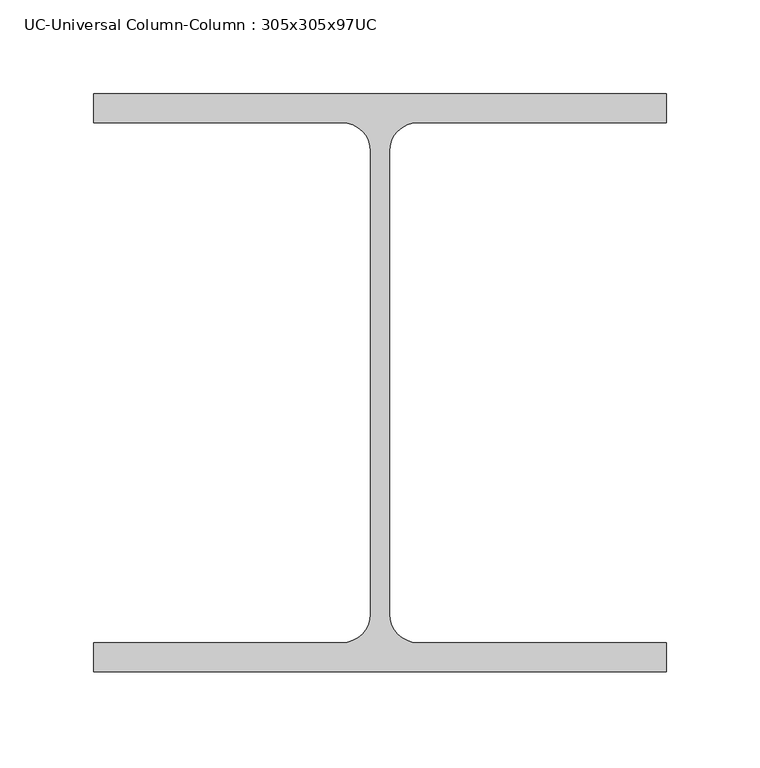
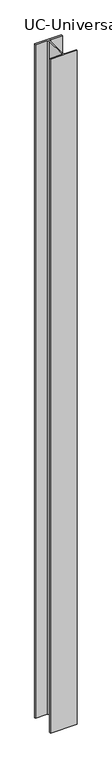
"""IFC4 building model written with IfcOpenShell, lengths in millimetres: column geometry, UC-Universal Column-Column : 305x305x97UC."""

import ifcopenshell
import ifcopenshell.guid

model = None  # the IFC model being written
_history = None  # IfcOwnerHistory: only IFC2X3 demands one
_inside = {}  # id of a spatial element -> (the spatial element, [elements in it])
_under = {}  # id of a project, library or spatial element -> (it, [spatial elements below it])
_declared = {}  # id of a project -> (the project, [libraries it declares])
_typed = {}  # id of a type object -> (the type object, [elements of that type])
_made_of = {}  # id of a material, layer set ... -> (it, [elements and type objects made of it])


def new_model(schema):
    """Start an empty IFC model of exactly this schema.

    Asked for "IFC4X3", IfcOpenShell would pick the latest addendum, in which some entities
    have other attributes; the version numbers below select the first issue.
    IFC2X3 requires an IfcOwnerHistory on every rooted entity: one is made here for all.
    """
    global model, _history
    if schema == "IFC4X3":
        model = ifcopenshell.file(schema_version=(4, 3, 0, 0))
    else:
        model = ifcopenshell.file(schema=schema)
    _inside.clear()
    _under.clear()
    _declared.clear()
    _typed.clear()
    _made_of.clear()
    _history = None
    if model.schema == "IFC2X3":
        org = make("IfcOrganization", Name="unknown")
        user = make(
            "IfcPersonAndOrganization",
            ThePerson=make("IfcPerson", FamilyName="unknown"),
            TheOrganization=org,
        )
        app = make(
            "IfcApplication",
            ApplicationDeveloper=org,
            Version="unknown",
            ApplicationFullName="unknown",
            ApplicationIdentifier="unknown",
        )
        _history = make(
            "IfcOwnerHistory",
            OwningUser=user,
            OwningApplication=app,
            ChangeAction="ADDED",
            CreationDate=0,
        )
    return model


def make(cls, **values):
    """One entity of the class cls with the attributes given. An attribute that is None is left unset."""
    return model.create_entity(
        cls, **{name: value for name, value in values.items() if value is not None}
    )


def rooted(cls, **values):
    """An entity with a GlobalId (a new one), such as an element, a storey or a relation."""
    return make(cls, GlobalId=ifcopenshell.guid.new(), OwnerHistory=_history, **values)


def si_unit(unit_type, name, prefix=None):
    """IfcSIUnit, for example si_unit("LENGTHUNIT", "METRE", prefix="MILLI")."""
    return make("IfcSIUnit", UnitType=unit_type, Prefix=prefix, Name=name)


def assignment(units):
    """IfcUnitAssignment: the units of a project."""
    return None if units is None else make("IfcUnitAssignment", Units=units)


def point(xyz):
    """IfcCartesianPoint."""
    return None if xyz is None else make("IfcCartesianPoint", Coordinates=xyz)


def direction(xyz):
    """IfcDirection."""
    return None if xyz is None else make("IfcDirection", DirectionRatios=xyz)


def frame(location, z_axis=None, x_axis=None):
    """IfcAxis2Placement3D, a coordinate frame: its origin and axes. An axis left out is left unset."""
    return make(
        "IfcAxis2Placement3D",
        Location=point(location),
        Axis=direction(z_axis),
        RefDirection=direction(x_axis),
    )


def frame_2d(location, x_axis=None):
    """IfcAxis2Placement2D, a coordinate frame in the plane: its origin and x axis."""
    return make(
        "IfcAxis2Placement2D", Location=point(location), RefDirection=direction(x_axis)
    )


def origin():
    """The frame at (0, 0, 0) with its axes left unset."""
    return frame((0.0, 0.0, 0.0))


def place(relative_to, where):
    """IfcLocalPlacement: puts the frame where relative to a parent placement (None: the world)."""
    return make(
        "IfcLocalPlacement", PlacementRelTo=relative_to, RelativePlacement=where
    )


def context(
    kind, dimensions, precision=None, world=None, true_north=None, identifier=None
):
    """IfcGeometricRepresentationContext, for example the 3D "Model" context."""
    return make(
        "IfcGeometricRepresentationContext",
        ContextIdentifier=identifier,
        ContextType=kind,
        CoordinateSpaceDimension=dimensions,
        Precision=precision,
        WorldCoordinateSystem=world,
        TrueNorth=true_north,
    )


def project(units=None, contexts=None):
    """IfcProject with its units and contexts."""
    return rooted(
        "IfcProject",
        Name="project",
        RepresentationContexts=contexts,
        UnitsInContext=assignment(units),
    )


def spatial(cls, under=None, at=None, **own):
    """A site, building, storey or space (cls), placed at a placement, below another one or the project."""
    s = rooted(cls, ObjectPlacement=at, **own)
    if under is not None:
        _under.setdefault(under.id(), (under, []))[1].append(s)
    return s


def polyline(points):
    """IfcPolyline through the points."""
    return make("IfcPolyline", Points=[point(p) for p in points])


def circle_curve(where, radius):
    """IfcCircle in the frame where."""
    return make("IfcCircle", Position=where, Radius=radius)


def trimmed(basis, trim1, trim2, sense, master):
    """IfcTrimmedCurve: the piece of a basis curve between two trims."""
    return make(
        "IfcTrimmedCurve",
        BasisCurve=basis,
        Trim1=trim1,
        Trim2=trim2,
        SenseAgreement=sense,
        MasterRepresentation=master,
    )


def segment(curve, same_sense, transition):
    """IfcCompositeCurveSegment."""
    return make(
        "IfcCompositeCurveSegment",
        Transition=transition,
        SameSense=same_sense,
        ParentCurve=curve,
    )


def composite_curve(segments, self_intersect=None):
    """IfcCompositeCurve: segments joined end to end."""
    return make("IfcCompositeCurve", Segments=segments, SelfIntersect=self_intersect)


def outline(outer, holes=None, kind="AREA"):
    """IfcArbitraryClosedProfileDef: a profile drawn as a closed curve; with holes, ...WithVoids."""
    if holes is None:
        return make("IfcArbitraryClosedProfileDef", ProfileType=kind, OuterCurve=outer)
    return make(
        "IfcArbitraryProfileDefWithVoids",
        ProfileType=kind,
        OuterCurve=outer,
        InnerCurves=holes,
    )


def extrude(swept, where, along, depth):
    """IfcExtrudedAreaSolid: the profile swept, set in the frame where, extruded along a direction by depth."""
    return make(
        "IfcExtrudedAreaSolid",
        SweptArea=swept,
        Position=where,
        ExtrudedDirection=direction(along),
        Depth=depth,
    )


def shape(context_of_items, identifier, shape_type, items):
    """IfcShapeRepresentation: the items that make up one representation, for example the "Body"."""
    return make(
        "IfcShapeRepresentation",
        ContextOfItems=context_of_items,
        RepresentationIdentifier=identifier,
        RepresentationType=shape_type,
        Items=items,
    )


def source(mapping_origin, context_of_items, identifier, shape_type, items):
    """IfcRepresentationMap: a shape defined once, which mapped items show again and again."""
    return make(
        "IfcRepresentationMap",
        MappingOrigin=mapping_origin,
        MappedRepresentation=shape(context_of_items, identifier, shape_type, items),
    )


def transform(
    local_origin,
    x_axis=None,
    y_axis=None,
    z_axis=None,
    scale=None,
    scale2=None,
    scale3=None,
    uniform=True,
):
    """IfcCartesianTransformationOperator3D, or its non-uniform kind. x_axis, y_axis, z_axis: its Axis1, 2, 3."""
    if uniform:
        return make(
            "IfcCartesianTransformationOperator3D",
            Axis1=direction(x_axis),
            Axis2=direction(y_axis),
            LocalOrigin=point(local_origin),
            Scale=scale,
            Axis3=direction(z_axis),
        )
    return make(
        "IfcCartesianTransformationOperator3DnonUniform",
        Axis1=direction(x_axis),
        Axis2=direction(y_axis),
        LocalOrigin=point(local_origin),
        Scale=scale,
        Axis3=direction(z_axis),
        Scale2=scale2,
        Scale3=scale3,
    )


def mapped(mapping_source, mapping_target):
    """IfcMappedItem: shows the shape of a source again, moved by a transform."""
    return make(
        "IfcMappedItem", MappingSource=mapping_source, MappingTarget=mapping_target
    )


def made_of(thing, what):
    """Note that an element or type object is made of a material, layer set ...; save() writes the relation."""
    if what is not None:
        _made_of.setdefault(what.id(), (what, []))[1].append(thing)
    return thing


def element(
    cls,
    number,
    at=None,
    inside=None,
    cuts=None,
    type_object=None,
    material=None,
    context=None,
    identifier="Body",
    shape_type=None,
    held_by="IfcProductDefinitionShape",
    body=None,
    shapes=None,
    **own,
):
    """One element of the class cls, such as IfcWall. Its Tag is "e" and its number.

    at: its placement. inside: the storey or other place that contains it. cuts: it is an
    opening in that element (IfcRelVoidsElement). A single representation is given by context,
    identifier, shape_type and body (its items); several are given by shapes. held_by: the class
    of the entity that holds the representations. save() writes the other relations.
    """
    e = rooted(cls, Tag="e%d" % number, ObjectPlacement=at, **own)
    if body is not None:
        shapes = [shape(context, identifier, shape_type, body)]
    if shapes is not None:
        e.Representation = make(held_by, Representations=shapes)
    if inside is not None:
        _inside.setdefault(inside.id(), (inside, []))[1].append(e)
    if cuts is not None:
        rooted(
            "IfcRelVoidsElement", RelatingBuildingElement=cuts, RelatedOpeningElement=e
        )
    if type_object is not None:
        _typed.setdefault(type_object.id(), (type_object, []))[1].append(e)
    return made_of(e, material)


def aggregate(whole, parts):
    """IfcRelAggregates: a whole, such as a stair, and the parts it consists of."""
    return rooted("IfcRelAggregates", RelatingObject=whole, RelatedObjects=parts)


def save(model, path):
    """Write the relations noted so far, then the file.

    IfcRelAggregates (storeys below a building ...), IfcRelContainedInSpatialStructure (elements
    in a storey), IfcRelDefinesByType, IfcRelAssociatesMaterial and IfcRelDeclares: one each for
    every whole, place, type object, material and project.
    """
    for whole, parts in _under.values():
        aggregate(whole, parts)
    for where, things in _inside.values():
        rooted(
            "IfcRelContainedInSpatialStructure",
            RelatedElements=things,
            RelatingStructure=where,
        )
    for kind, things in _typed.values():
        rooted("IfcRelDefinesByType", RelatedObjects=things, RelatingType=kind)
    for what, things in _made_of.values():
        rooted("IfcRelAssociatesMaterial", RelatedObjects=things, RelatingMaterial=what)
    for by, libraries in _declared.values():
        rooted("IfcRelDeclares", RelatingContext=by, RelatedDefinitions=libraries)
    model.write(path)


def uc_universal_column_column_305x305x97uc_43a052ce(model_context):
    return source(origin(), model_context, "Body", "SweptSolid", [
        extrude(outline(composite_curve([segment(polyline([(152.65, 153.95), (152.65, 138.55), (20.15, 138.55)]), True, "CONTINUOUS"), segment(trimmed(circle_curve(frame_2d((20.15, 123.35)), 15.2), [point((20.15, 138.55))], [point((4.95, 123.35))], True, "CARTESIAN"), True, "CONTINUOUS"), segment(polyline([(4.95, 123.35), (4.95, -123.35)]), True, "CONTINUOUS"), segment(trimmed(circle_curve(frame_2d((20.15, -123.35)), 15.2), [point((4.95, -123.35))], [point((20.15, -138.55))], True, "CARTESIAN"), True, "CONTINUOUS"), segment(polyline([(20.15, -138.55), (152.65, -138.55), (152.65, -153.95), (-152.65, -153.95), (-152.65, -138.55), (-20.15, -138.55)]), True, "CONTINUOUS"), segment(trimmed(circle_curve(frame_2d((-20.15, -123.35)), 15.2), [point((-20.15, -138.55))], [point((-4.95, -123.35))], True, "CARTESIAN"), True, "CONTINUOUS"), segment(polyline([(-4.95, -123.35), (-4.95, 123.35)]), True, "CONTINUOUS"), segment(trimmed(circle_curve(frame_2d((-20.15, 123.35)), 15.2), [point((-4.95, 123.35))], [point((-20.15, 138.55))], True, "CARTESIAN"), True, "CONTINUOUS"), segment(polyline([(-20.15, 138.55), (-152.65, 138.55), (-152.65, 153.95), (152.65, 153.95)]), True, "CONTINUOUS")], self_intersect=False)), frame((0.0, 0.0, -1500.0), z_axis=(0.0, 0.0, 1.0), x_axis=(1.0, 0.0, 0.0)), (0.0, 0.0, 1.0), 8100.0),
    ])


if __name__ == "__main__":
    model = new_model("IFC4")
    model_context = context("Model", 3, world=origin())
    ifc_project = project(units=[si_unit("LENGTHUNIT", "METRE", prefix="MILLI")], contexts=[model_context])
    site = spatial("IfcSite", under=ifc_project)
    building = spatial("IfcBuilding", under=site)
    placement = place(None, origin())
    uc_universal_column_column_305x305x97uc_shape = uc_universal_column_column_305x305x97uc_43a052ce(model_context)
    element("IfcColumn", 1, ObjectType="UC-Universal Column-Column : 305x305x97UC", at=placement, inside=building, context=model_context, shape_type="MappedRepresentation", body=[
        mapped(uc_universal_column_column_305x305x97uc_shape, transform((0.0, 0.0, 0.0), x_axis=(1.0, 0.0, 0.0), y_axis=(0.0, 1.0, 0.0), z_axis=(0.0, 0.0, 1.0))),
    ])
    save(model, "model.ifc")

# Revit data of these elements
# Type "UC-Universal Column-Column : 305x305x97UC"
#   Keynote = "G10"
#   Nominal h = ""
#   W = 0
#   Ix = 0
#   M = 96.9
#   Zx = 0
#   b = 305.3 mm
#   h = 307.9 mm
#   r = 15.2 mm
#   s = 9.9 mm
#   t = 15.4 mm
#   A = 123 m²
#   Structural Material [instance default] = Steel, 45-345
#   Assembly Code = ""
# Element 1 (IfcColumn, "UC-Universal Column-Column : 305x305x97UC")
#   Materials on its faces: "Steel, 45-345"
# Materials
#   "Steel, 45-345": class "Metal", colour RGB 247 247 247, transparency 0, Description = "Steel 345 MPa", Cost = 0
